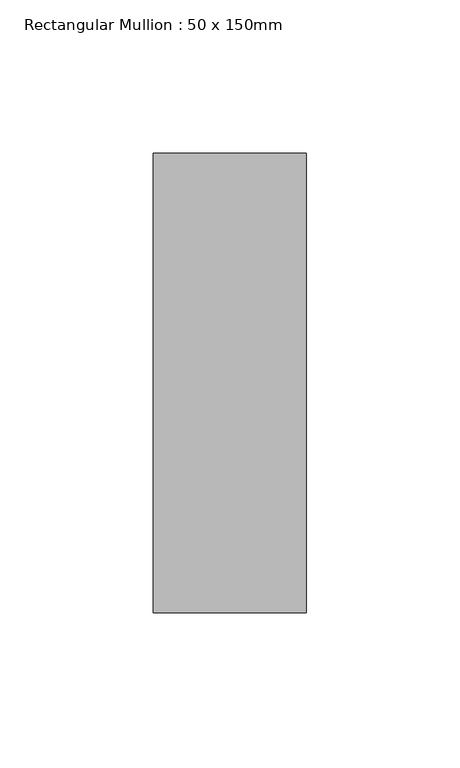
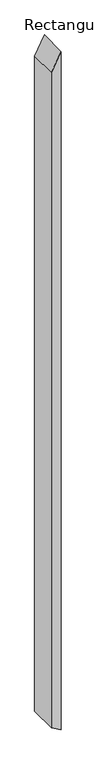
"""IFC4 building model written with IfcOpenShell, lengths in millimetres: member geometry, Rectangular Mullion : 50 x 150mm."""

from ifc_helpers import new_model, si_unit, frame, origin, place, context, project, spatial, polyline, outline, extrude, source, transform, mapped, element, save


def rectangular_mullion_50_x_150mm_c12f4f4b(model_context):
    return source(origin(), model_context, "Body", "SweptSolid", [
        extrude(outline(polyline([(0.0, 0.0), (-98.1080667, -50.0), (-3682.0310611, -50.0), (-3710.9535778, 0.0), (0.0, 0.0)])), frame((0.0, -75.0, 0.0), z_axis=(0.0, 1.0, 0.0), x_axis=(0.0, 0.0, 1.0)), (0.0, 0.0, 1.0), 150.0),
    ])


if __name__ == "__main__":
    model = new_model("IFC4")
    model_context = context("Model", 3, world=origin())
    ifc_project = project(units=[si_unit("LENGTHUNIT", "METRE", prefix="MILLI")], contexts=[model_context])
    site = spatial("IfcSite", under=ifc_project)
    building = spatial("IfcBuilding", under=site)
    placement = place(None, origin())
    rectangular_mullion_50_x_150mm_shape = rectangular_mullion_50_x_150mm_c12f4f4b(model_context)
    element("IfcMember", 1, ObjectType="Rectangular Mullion : 50 x 150mm", at=placement, inside=building, context=model_context, shape_type="MappedRepresentation", body=[
        mapped(rectangular_mullion_50_x_150mm_shape, transform((0.0, 0.0, 0.0), x_axis=(1.0, 0.0, 0.0), y_axis=(0.0, 1.0, 0.0), z_axis=(0.0, 0.0, 1.0))),
    ])
    save(model, "model.ifc")

# Revit data of these elements
# Type "Rectangular Mullion : 50 x 150mm"
#   built-in parameter 1007304 = 0.492126 (stored number, unit not read)
#   built-in parameter 1007301 = 0.082021 (stored number, unit not read)
#   built-in parameter 1007300 = 0.082021 (stored number, unit not read)
# Element 1 (IfcMember, "Rectangular Mullion : 50 x 150mm")
#   Materials on its faces: "Metal - Aluminium"
# Materials
#   "Metal - Aluminium": class "Metal", colour RGB 247 247 247, transparency 0
